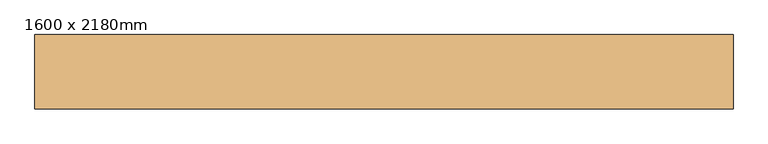
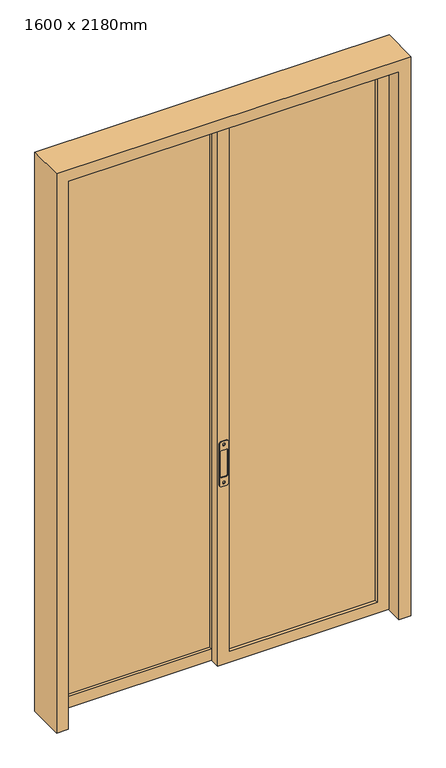
"""IFC4 building model written with IfcOpenShell, lengths in millimetres: door geometry, Porta de correr dupla envidraçada sem revestimento : 1600 x 2180mm."""

from ifc_helpers import new_model, si_unit, point, frame, frame_2d, origin, place, context, project, spatial, polyline, circle_curve, trimmed, segment, composite_curve, outline, extrude, source, transform, mapped, element, save


def door_1600_x_2180mm_53dcaf88(model_context):
    return source(origin(), model_context, "Body", "SweptSolid", [
        extrude(outline(composite_curve([segment(trimmed(circle_curve(frame_2d((990.0, -10.0)), 10.0), [point((1000.0, -10.0))], [point((990.0, -20.0))], False, "CARTESIAN"), True, "CONTINUOUS"), segment(polyline([(990.0, -20.0), (810.0, -20.0)]), True, "CONTINUOUS"), segment(trimmed(circle_curve(frame_2d((810.0, -10.0)), 10.0), [point((810.0, -20.0))], [point((800.0, -10.0))], False, "CARTESIAN"), True, "CONTINUOUS"), segment(polyline([(800.0, -10.0), (800.0, 10.0)]), True, "CONTINUOUS"), segment(trimmed(circle_curve(frame_2d((810.0, 10.0)), 10.0), [point((800.0, 10.0))], [point((810.0, 20.0))], False, "CARTESIAN"), True, "CONTINUOUS"), segment(polyline([(810.0, 20.0), (990.0, 20.0)]), True, "CONTINUOUS"), segment(trimmed(circle_curve(frame_2d((990.0, 10.0)), 10.0), [point((990.0, 20.0))], [point((1000.0, 10.0))], False, "CARTESIAN"), True, "CONTINUOUS"), segment(polyline([(1000.0, 10.0), (1000.0, -10.0)]), True, "CONTINUOUS")], self_intersect=False), holes=[composite_curve([segment(polyline([(960.0, -10.0), (960.0, 10.0)]), True, "CONTINUOUS"), segment(trimmed(circle_curve(frame_2d((955.0, 10.0)), 5.0), [point((960.0, 10.0))], [point((955.0, 15.0))], True, "CARTESIAN"), True, "CONTINUOUS"), segment(polyline([(955.0, 15.0), (845.0, 15.0)]), True, "CONTINUOUS"), segment(trimmed(circle_curve(frame_2d((845.0, 10.0)), 5.0), [point((845.0, 15.0))], [point((840.0, 10.0))], True, "CARTESIAN"), True, "CONTINUOUS"), segment(polyline([(840.0, 10.0), (840.0, -10.0)]), True, "CONTINUOUS"), segment(trimmed(circle_curve(frame_2d((845.0, -10.0)), 5.0), [point((840.0, -10.0))], [point((845.0, -15.0))], True, "CARTESIAN"), True, "CONTINUOUS"), segment(polyline([(845.0, -15.0), (955.0, -15.0)]), True, "CONTINUOUS"), segment(trimmed(circle_curve(frame_2d((955.0, -10.0)), 5.0), [point((955.0, -15.0))], [point((960.0, -10.0))], True, "CARTESIAN"), True, "CONTINUOUS")], self_intersect=False), composite_curve([segment(trimmed(circle_curve(frame_2d((985.0, 0.0)), 5.0), [point((985.0, -5.0))], [point((985.0, 5.0))], True, "CARTESIAN"), True, "CONTINUOUS"), segment(trimmed(circle_curve(frame_2d((985.0, 0.0)), 5.0), [point((985.0, 5.0))], [point((985.0, -5.0))], True, "CARTESIAN"), True, "CONTINUOUS")], self_intersect=False), composite_curve([segment(trimmed(circle_curve(frame_2d((815.0, 0.0)), 5.0), [point((815.0, -5.0))], [point((815.0, 5.0))], True, "CARTESIAN"), True, "CONTINUOUS"), segment(trimmed(circle_curve(frame_2d((815.0, 0.0)), 5.0), [point((815.0, 5.0))], [point((815.0, -5.0))], True, "CARTESIAN"), True, "CONTINUOUS")], self_intersect=False)]), frame((0.0, -8.4, 0.0), z_axis=(0.0, 1.0, 0.0), x_axis=(0.0, 0.0, 1.0)), (0.0, 0.0, 1.0), 3.0),
        extrude(outline(polyline([(2450.0, 25.0), (2450.0, -700.0), (0.0, -700.0), (0.0, 25.0), (2450.0, 25.0)]), holes=[polyline([(2400.0, -650.0), (2400.0, -25.0), (50.0, -25.0), (50.0, -650.0), (2400.0, -650.0)])]), frame((0.0, 39.6, 0.0), z_axis=(0.0, 1.0, 0.0), x_axis=(0.0, 0.0, 1.0)), (0.0, 0.0, 1.0), 40.0),
        extrude(outline(polyline([(2450.0, 700.0), (2450.0, -25.0), (0.0, -25.0), (0.0, 700.0), (2450.0, 700.0)]), holes=[polyline([(2400.0, 25.0), (2400.0, 650.0), (50.0, 650.0), (50.0, 25.0), (2400.0, 25.0)])]), frame((0.0, -5.4, 0.0), z_axis=(0.0, 1.0, 0.0), x_axis=(0.0, 0.0, 1.0)), (0.0, 0.0, 1.0), 40.0),
        extrude(outline(polyline([(0.0, 750.0), (2500.0, 750.0), (2500.0, -750.0), (0.0, -750.0), (0.0, -700.0), (2450.0, -700.0), (2450.0, 700.0), (0.0, 700.0), (0.0, 750.0)])), frame((0.0, -79.6, 0.0), z_axis=(0.0, 1.0, 0.0), x_axis=(0.0, 0.0, 1.0)), (0.0, 0.0, 1.0), 159.2),
        extrude(outline(polyline([(-25.0, 52.6), (-650.0, 52.6), (-650.0, 66.6), (-25.0, 66.6), (-25.0, 52.6)])), frame((0.0, 0.0, 50.0), z_axis=(0.0, 0.0, 1.0), x_axis=(1.0, 0.0, 0.0)), (0.0, 0.0, 1.0), 2350.0),
        extrude(outline(polyline([(650.0, 7.6), (25.0, 7.6), (25.0, 21.6), (650.0, 21.6), (650.0, 7.6)])), frame((0.0, 0.0, 50.0), z_axis=(0.0, 0.0, 1.0), x_axis=(1.0, 0.0, 0.0)), (0.0, 0.0, 1.0), 2350.0),
        extrude(outline(polyline([(-650.0, 52.6), (-650.0, 66.6), (-25.0, 66.6), (-25.0, 52.6), (-650.0, 52.6)])), frame((0.0, 0.0, 50.0), z_axis=(0.0, 0.0, 1.0), x_axis=(1.0, 0.0, 0.0)), (0.0, 0.0, 1.0), 2350.0),
        extrude(outline(polyline([(650.0, 7.6), (25.0, 7.6), (25.0, 21.6), (650.0, 21.6), (650.0, 7.6)])), frame((0.0, 0.0, 50.0), z_axis=(0.0, 0.0, 1.0), x_axis=(1.0, 0.0, 0.0)), (0.0, 0.0, 1.0), 2350.0),
    ])


if __name__ == "__main__":
    model = new_model("IFC4")
    model_context = context("Model", 3, world=origin())
    ifc_project = project(units=[si_unit("LENGTHUNIT", "METRE", prefix="MILLI")], contexts=[model_context])
    site = spatial("IfcSite", under=ifc_project)
    building = spatial("IfcBuilding", under=site)
    placement = place(None, origin())
    door_1600_x_2180mm_shape = door_1600_x_2180mm_53dcaf88(model_context)
    element("IfcDoor", 1, ObjectType="Porta de correr dupla envidraçada sem revestimento : 1600 x 2180mm", at=placement, inside=building, context=model_context, shape_type="MappedRepresentation", body=[
        mapped(door_1600_x_2180mm_shape, transform((0.0, 0.0, 0.0), x_axis=(1.0, 0.0, 0.0), y_axis=(0.0, 1.0, 0.0), z_axis=(0.0, 0.0, 1.0))),
    ])
    save(model, "model.ifc")

# Revit data of these elements
# Type "Porta de correr dupla envidraçada sem revestimento : 1600 x 2180mm"
#   Type Mark = "P56"
#   Construction Type Id = "GSP4R"
#   Analytic Construction = "Vidraça única Pilkington 1/8 pol"
#   Visual Light Transmittance = 0.9
#   Thickness = 0.09 m
#   Solar Heat Gain Coefficient = 0.78
#   Rough Width = 1.50 m
#   Rough Height = 2.50 m
#   Largura da moldura do painel = 0.05 m
#   Espessura da moldura do painel = 0.04 m
#   Heat Transfer Coefficient (U) = 3.6886 W/(m²·K)
#   Largura da maçaneta = 0.04 m
#   Altura do puxador = 0.20 m
#   Largura da estrutura = 0.05 m
#   Height = 2.50 m
#   Width = 1.50 m
#   Function = 1
#   Material do puxador = none
#   Vidro = Vidro - Janela
#   Material da estrutura = Aluminum Sill
#   Wall Closure = (empty or 0)
# Element 1 (IfcDoor, "Porta de correr dupla envidraçada sem revestimento : 1600 x 2180mm")
#   Materials on its faces: "Aluminum Sill", "Vidro - Janela"
# Materials
#   "Vidro - Janela": class "Vidro", colour RGB 249 249 249, transparency 1, Cost = 0
#   "Aluminum Sill": class "Não atribuído", colour RGB 247 247 247, transparency 0
